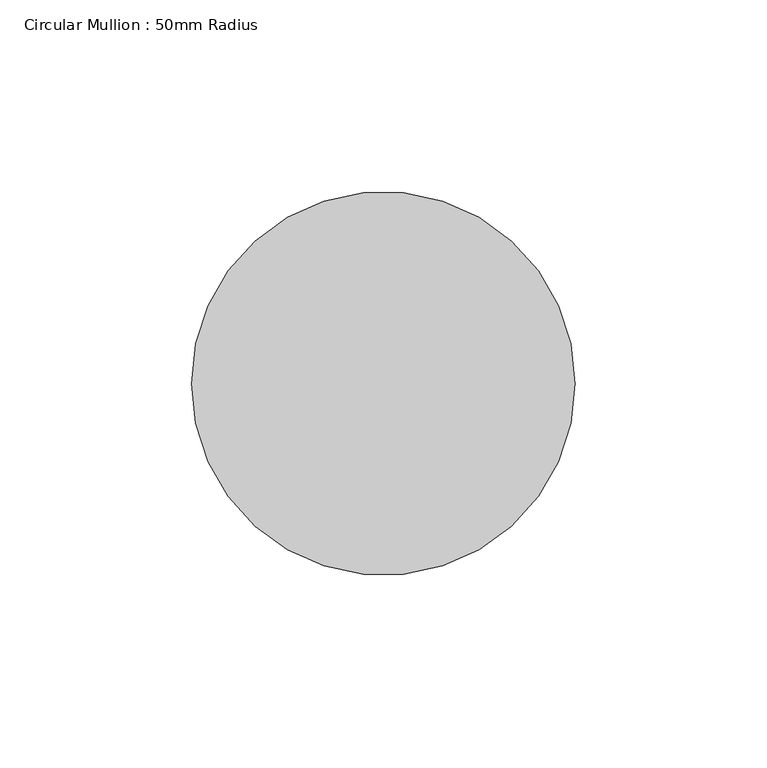
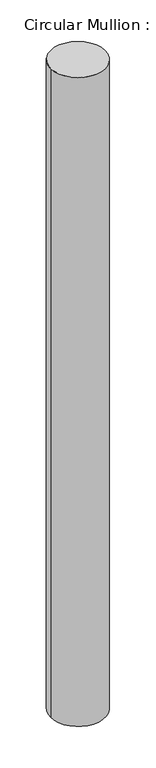
"""IFC4 building model written with IfcOpenShell, lengths in millimetres: member geometry, Circular Mullion : 50mm Radius."""

from ifc_helpers import new_model, si_unit, point, frame, origin, origin_2d, place, context, project, spatial, circle_curve, trimmed, segment, composite_curve, outline, extrude, source, transform, mapped, element, save


def circular_mullion_50mm_radius_e9cb4ea8(model_context):
    return source(origin(), model_context, "Body", "SweptSolid", [
        extrude(outline(composite_curve([segment(trimmed(circle_curve(origin_2d(), 50.0), [point((50.0, 0.0))], [point((-50.0, 0.0))], False, "CARTESIAN"), True, "CONTINUOUS"), segment(trimmed(circle_curve(origin_2d(), 50.0), [point((-50.0, 0.0))], [point((50.0, 0.0))], False, "CARTESIAN"), True, "CONTINUOUS")], self_intersect=False)), frame((0.0, 0.0, -1260.5321842), z_axis=(0.0, 0.0, 1.0), x_axis=(1.0, 0.0, 0.0)), (0.0, 0.0, 1.0), 1260.5321842),
    ])


if __name__ == "__main__":
    model = new_model("IFC4")
    model_context = context("Model", 3, world=origin())
    ifc_project = project(units=[si_unit("LENGTHUNIT", "METRE", prefix="MILLI")], contexts=[model_context])
    site = spatial("IfcSite", under=ifc_project)
    building = spatial("IfcBuilding", under=site)
    placement = place(None, origin())
    circular_mullion_50mm_radius_shape = circular_mullion_50mm_radius_e9cb4ea8(model_context)
    element("IfcMember", 1, ObjectType="Circular Mullion : 50mm Radius", at=placement, inside=building, context=model_context, shape_type="MappedRepresentation", body=[
        mapped(circular_mullion_50mm_radius_shape, transform((0.0, 0.0, 0.0), x_axis=(1.0, 0.0, 0.0), y_axis=(0.0, 1.0, 0.0), z_axis=(0.0, 0.0, 1.0))),
    ])
    save(model, "model.ifc")

# Revit data of these elements
# Type "Circular Mullion : 50mm Radius"
#   built-in parameter 1007350 = 0.164042 (stored number, unit not read)
# Element 1 (IfcMember, "Circular Mullion : 50mm Radius")
#   Materials on its faces: "Aluminium"
# Materials
#   "Aluminium": class "Metal", colour RGB 247 247 247, transparency 0, Description = "Aluminium 6061", Cost = 0
